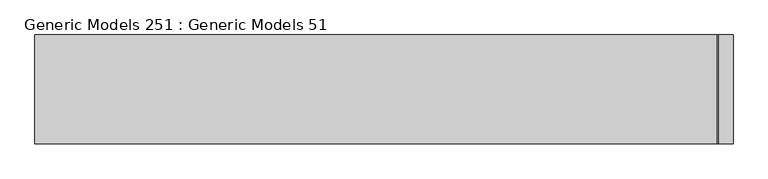
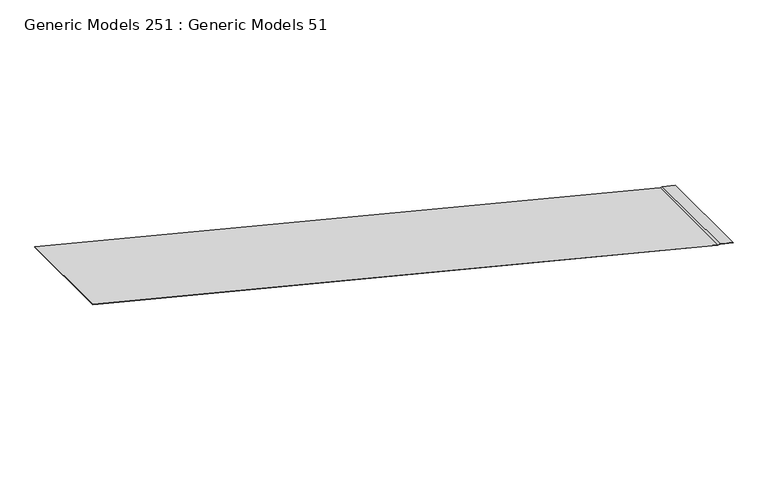
"""IFC4 building model written with IfcOpenShell, lengths in millimetres: proxy geometry, Generic Models 251 : Generic Models 51."""

from ifc_helpers import new_model, si_unit, frame, origin, place, context, project, spatial, polyline, outline, extrude, source, transform, mapped, element, save


def generic_models_251_generic_models_51_c5c024df(model_context):
    return source(origin(), model_context, "Body", "SweptSolid", [
        extrude(outline(polyline([(127216.8299763, -31486.9130721), (127693.2660617, -33392.6574136), (127692.4960111, -33392.8499262), (127216.0100736, -31486.9061762), (127217.7105327, -31480.5599764), (127207.8465158, -31441.1039086), (127208.6165664, -31440.911396), (127218.5304354, -31480.5668722), (127216.8299763, -31486.9130721)])), frame((0.0, 21665.9639348, 0.0), z_axis=(0.0, 1.0, 0.0), x_axis=(0.0, 0.0, 1.0)), (0.0, 0.0, 1.0), 304.8),
    ])


if __name__ == "__main__":
    model = new_model("IFC4")
    model_context = context("Model", 3, world=origin())
    ifc_project = project(units=[si_unit("LENGTHUNIT", "METRE", prefix="MILLI")], contexts=[model_context])
    site = spatial("IfcSite", under=ifc_project)
    building = spatial("IfcBuilding", under=site)
    placement = place(None, origin())
    generic_models_251_generic_models_51_shape = generic_models_251_generic_models_51_c5c024df(model_context)
    element("IfcBuildingElementProxy", 1, Name="Generic Models 251 : Generic Models 51", ObjectType="Generic Models 251 : Generic Models 51", at=placement, inside=building, context=model_context, shape_type="MappedRepresentation", body=[
        mapped(generic_models_251_generic_models_51_shape, transform((0.0, 0.0, 0.0), x_axis=(1.0, 0.0, 0.0), y_axis=(0.0, 1.0, 0.0), z_axis=(0.0, 0.0, 1.0))),
    ])
    save(model, "model.ifc")

# Revit data of these elements
# Element 1 (IfcBuildingElementProxy, "Generic Models 251 : Generic Models 51")
#   Materials on its faces: "_(2) LAYERS NO. 30 ASTM D226 ASPHALT SATURATED ORGANIC FELT @ ROOF"
# Materials
#   "_(2) LAYERS NO. 30 ASTM D226 ASPHALT SATURATED ORGANIC FELT @ ROOF": class "Generic", colour RGB 67 154 161, transparency 0, Cost = 0
